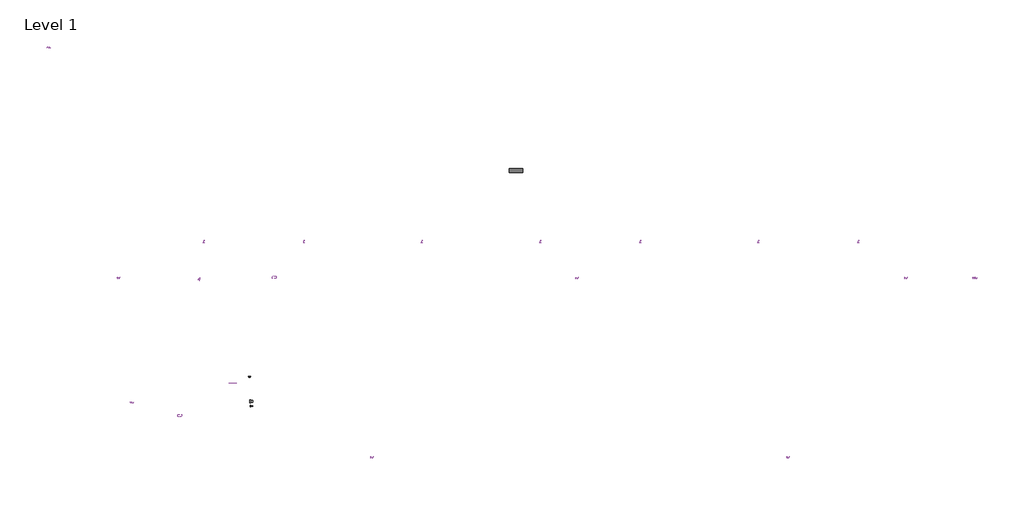
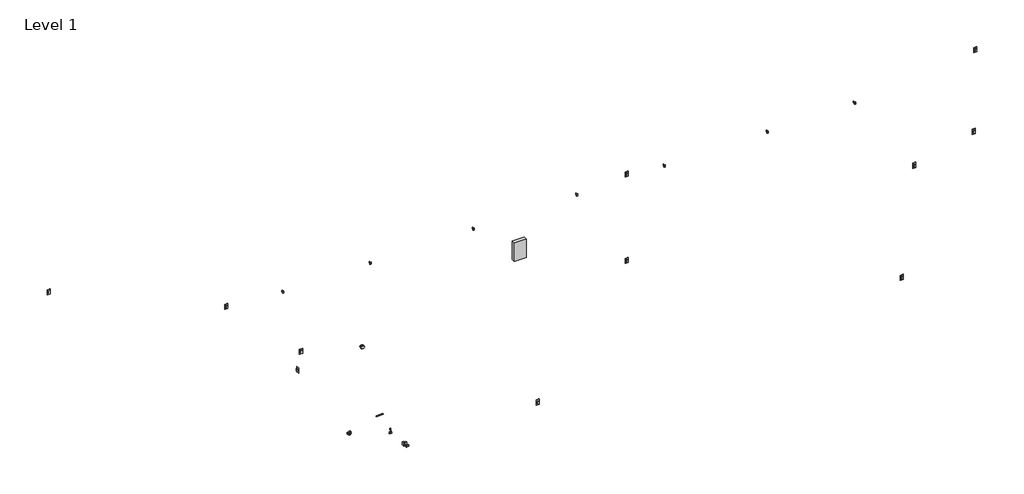
# One storey: 26 proxies.
"""IFC4 building model written with IfcOpenShell, lengths in millimetres."""

import ifcopenshell
import ifcopenshell.guid

model = None  # the IFC model being written
_history = None  # IfcOwnerHistory: only IFC2X3 demands one
_inside = {}  # id of a spatial element -> (the spatial element, [elements in it])
_under = {}  # id of a project, library or spatial element -> (it, [spatial elements below it])
_declared = {}  # id of a project -> (the project, [libraries it declares])
_typed = {}  # id of a type object -> (the type object, [elements of that type])
_made_of = {}  # id of a material, layer set ... -> (it, [elements and type objects made of it])


def new_model(schema):
    """Start an empty IFC model of exactly this schema.

    Asked for "IFC4X3", IfcOpenShell would pick the latest addendum, in which some entities
    have other attributes; the version numbers below select the first issue.
    IFC2X3 requires an IfcOwnerHistory on every rooted entity: one is made here for all.
    """
    global model, _history
    if schema == "IFC4X3":
        model = ifcopenshell.file(schema_version=(4, 3, 0, 0))
    else:
        model = ifcopenshell.file(schema=schema)
    _inside.clear()
    _under.clear()
    _declared.clear()
    _typed.clear()
    _made_of.clear()
    _history = None
    if model.schema == "IFC2X3":
        org = make("IfcOrganization", Name="unknown")
        user = make(
            "IfcPersonAndOrganization",
            ThePerson=make("IfcPerson", FamilyName="unknown"),
            TheOrganization=org,
        )
        app = make(
            "IfcApplication",
            ApplicationDeveloper=org,
            Version="unknown",
            ApplicationFullName="unknown",
            ApplicationIdentifier="unknown",
        )
        _history = make(
            "IfcOwnerHistory",
            OwningUser=user,
            OwningApplication=app,
            ChangeAction="ADDED",
            CreationDate=0,
        )
    return model


def make(cls, **values):
    """One entity of the class cls with the attributes given. An attribute that is None is left unset."""
    return model.create_entity(
        cls, **{name: value for name, value in values.items() if value is not None}
    )


def rooted(cls, **values):
    """An entity with a GlobalId (a new one), such as an element, a storey or a relation."""
    return make(cls, GlobalId=ifcopenshell.guid.new(), OwnerHistory=_history, **values)


def si_unit(unit_type, name, prefix=None):
    """IfcSIUnit, for example si_unit("LENGTHUNIT", "METRE", prefix="MILLI")."""
    return make("IfcSIUnit", UnitType=unit_type, Prefix=prefix, Name=name)


def assignment(units):
    """IfcUnitAssignment: the units of a project."""
    return None if units is None else make("IfcUnitAssignment", Units=units)


def point(xyz):
    """IfcCartesianPoint."""
    return None if xyz is None else make("IfcCartesianPoint", Coordinates=xyz)


def direction(xyz):
    """IfcDirection."""
    return None if xyz is None else make("IfcDirection", DirectionRatios=xyz)


def frame(location, z_axis=None, x_axis=None):
    """IfcAxis2Placement3D, a coordinate frame: its origin and axes. An axis left out is left unset."""
    return make(
        "IfcAxis2Placement3D",
        Location=point(location),
        Axis=direction(z_axis),
        RefDirection=direction(x_axis),
    )


def frame_2d(location, x_axis=None):
    """IfcAxis2Placement2D, a coordinate frame in the plane: its origin and x axis."""
    return make(
        "IfcAxis2Placement2D", Location=point(location), RefDirection=direction(x_axis)
    )


def origin():
    """The frame at (0, 0, 0) with its axes left unset."""
    return frame((0.0, 0.0, 0.0))


def origin_with_axes():
    """The frame at (0, 0, 0) with the z axis (0, 0, 1) and the x axis (1, 0, 0) written out."""
    return frame((0.0, 0.0, 0.0), z_axis=(0.0, 0.0, 1.0), x_axis=(1.0, 0.0, 0.0))


def origin_2d():
    """The frame at (0, 0) in the plane with its x axis left unset."""
    return frame_2d((0.0, 0.0))


def place(relative_to, where):
    """IfcLocalPlacement: puts the frame where relative to a parent placement (None: the world)."""
    return make(
        "IfcLocalPlacement", PlacementRelTo=relative_to, RelativePlacement=where
    )


def context(
    kind, dimensions, precision=None, world=None, true_north=None, identifier=None
):
    """IfcGeometricRepresentationContext, for example the 3D "Model" context."""
    return make(
        "IfcGeometricRepresentationContext",
        ContextIdentifier=identifier,
        ContextType=kind,
        CoordinateSpaceDimension=dimensions,
        Precision=precision,
        WorldCoordinateSystem=world,
        TrueNorth=true_north,
    )


def project(units=None, contexts=None):
    """IfcProject with its units and contexts."""
    return rooted(
        "IfcProject",
        Name="project",
        RepresentationContexts=contexts,
        UnitsInContext=assignment(units),
    )


def spatial(cls, under=None, at=None, **own):
    """A site, building, storey or space (cls), placed at a placement, below another one or the project."""
    s = rooted(cls, ObjectPlacement=at, **own)
    if under is not None:
        _under.setdefault(under.id(), (under, []))[1].append(s)
    return s


def polyline(points):
    """IfcPolyline through the points."""
    return make("IfcPolyline", Points=[point(p) for p in points])


def circle_curve(where, radius):
    """IfcCircle in the frame where."""
    return make("IfcCircle", Position=where, Radius=radius)


def ellipse_curve(where, semi_axis1, semi_axis2):
    """IfcEllipse in the frame where."""
    return make(
        "IfcEllipse", Position=where, SemiAxis1=semi_axis1, SemiAxis2=semi_axis2
    )


def trimmed(basis, trim1, trim2, sense, master):
    """IfcTrimmedCurve: the piece of a basis curve between two trims."""
    return make(
        "IfcTrimmedCurve",
        BasisCurve=basis,
        Trim1=trim1,
        Trim2=trim2,
        SenseAgreement=sense,
        MasterRepresentation=master,
    )


def segment(curve, same_sense, transition):
    """IfcCompositeCurveSegment."""
    return make(
        "IfcCompositeCurveSegment",
        Transition=transition,
        SameSense=same_sense,
        ParentCurve=curve,
    )


def composite_curve(segments, self_intersect=None):
    """IfcCompositeCurve: segments joined end to end."""
    return make("IfcCompositeCurve", Segments=segments, SelfIntersect=self_intersect)


def outline(outer, holes=None, kind="AREA"):
    """IfcArbitraryClosedProfileDef: a profile drawn as a closed curve; with holes, ...WithVoids."""
    if holes is None:
        return make("IfcArbitraryClosedProfileDef", ProfileType=kind, OuterCurve=outer)
    return make(
        "IfcArbitraryProfileDefWithVoids",
        ProfileType=kind,
        OuterCurve=outer,
        InnerCurves=holes,
    )


def extrude(swept, where, along, depth):
    """IfcExtrudedAreaSolid: the profile swept, set in the frame where, extruded along a direction by depth."""
    return make(
        "IfcExtrudedAreaSolid",
        SweptArea=swept,
        Position=where,
        ExtrudedDirection=direction(along),
        Depth=depth,
    )


def shape(context_of_items, identifier, shape_type, items):
    """IfcShapeRepresentation: the items that make up one representation, for example the "Body"."""
    return make(
        "IfcShapeRepresentation",
        ContextOfItems=context_of_items,
        RepresentationIdentifier=identifier,
        RepresentationType=shape_type,
        Items=items,
    )


def source(mapping_origin, context_of_items, identifier, shape_type, items):
    """IfcRepresentationMap: a shape defined once, which mapped items show again and again."""
    return make(
        "IfcRepresentationMap",
        MappingOrigin=mapping_origin,
        MappedRepresentation=shape(context_of_items, identifier, shape_type, items),
    )


def transform(
    local_origin,
    x_axis=None,
    y_axis=None,
    z_axis=None,
    scale=None,
    scale2=None,
    scale3=None,
    uniform=True,
):
    """IfcCartesianTransformationOperator3D, or its non-uniform kind. x_axis, y_axis, z_axis: its Axis1, 2, 3."""
    if uniform:
        return make(
            "IfcCartesianTransformationOperator3D",
            Axis1=direction(x_axis),
            Axis2=direction(y_axis),
            LocalOrigin=point(local_origin),
            Scale=scale,
            Axis3=direction(z_axis),
        )
    return make(
        "IfcCartesianTransformationOperator3DnonUniform",
        Axis1=direction(x_axis),
        Axis2=direction(y_axis),
        LocalOrigin=point(local_origin),
        Scale=scale,
        Axis3=direction(z_axis),
        Scale2=scale2,
        Scale3=scale3,
    )


def mapped(mapping_source, mapping_target):
    """IfcMappedItem: shows the shape of a source again, moved by a transform."""
    return make(
        "IfcMappedItem", MappingSource=mapping_source, MappingTarget=mapping_target
    )


def made_of(thing, what):
    """Note that an element or type object is made of a material, layer set ...; save() writes the relation."""
    if what is not None:
        _made_of.setdefault(what.id(), (what, []))[1].append(thing)
    return thing


def element(
    cls,
    number,
    at=None,
    inside=None,
    cuts=None,
    type_object=None,
    material=None,
    context=None,
    identifier="Body",
    shape_type=None,
    held_by="IfcProductDefinitionShape",
    body=None,
    shapes=None,
    **own,
):
    """One element of the class cls, such as IfcWall. Its Tag is "e" and its number.

    at: its placement. inside: the storey or other place that contains it. cuts: it is an
    opening in that element (IfcRelVoidsElement). A single representation is given by context,
    identifier, shape_type and body (its items); several are given by shapes. held_by: the class
    of the entity that holds the representations. save() writes the other relations.
    """
    e = rooted(cls, Tag="e%d" % number, ObjectPlacement=at, **own)
    if body is not None:
        shapes = [shape(context, identifier, shape_type, body)]
    if shapes is not None:
        e.Representation = make(held_by, Representations=shapes)
    if inside is not None:
        _inside.setdefault(inside.id(), (inside, []))[1].append(e)
    if cuts is not None:
        rooted(
            "IfcRelVoidsElement", RelatingBuildingElement=cuts, RelatedOpeningElement=e
        )
    if type_object is not None:
        _typed.setdefault(type_object.id(), (type_object, []))[1].append(e)
    return made_of(e, material)


def aggregate(whole, parts):
    """IfcRelAggregates: a whole, such as a stair, and the parts it consists of."""
    return rooted("IfcRelAggregates", RelatingObject=whole, RelatedObjects=parts)


def save(model, path):
    """Write the relations noted so far, then the file.

    IfcRelAggregates (storeys below a building ...), IfcRelContainedInSpatialStructure (elements
    in a storey), IfcRelDefinesByType, IfcRelAssociatesMaterial and IfcRelDeclares: one each for
    every whole, place, type object, material and project.
    """
    for whole, parts in _under.values():
        aggregate(whole, parts)
    for where, things in _inside.values():
        rooted(
            "IfcRelContainedInSpatialStructure",
            RelatedElements=things,
            RelatingStructure=where,
        )
    for kind, things in _typed.values():
        rooted("IfcRelDefinesByType", RelatedObjects=things, RelatingType=kind)
    for what, things in _made_of.values():
        rooted("IfcRelAssociatesMaterial", RelatedObjects=things, RelatingMaterial=what)
    for by, libraries in _declared.values():
        rooted("IfcRelDeclares", RelatingContext=by, RelatedDefinitions=libraries)
    model.write(path)


def plane_surface(at):
    """IfcPlane: the flat surface through the origin of the frame at, square to its z axis."""
    return make("IfcPlane", Position=at)


def cylinder_surface(at, radius):
    """IfcCylindricalSurface: all points at the distance radius from the z axis of the frame at."""
    return make("IfcCylindricalSurface", Position=at, Radius=radius)


def revolved_surface(curve, axis_point, axis_direction):
    """IfcSurfaceOfRevolution: the curve turned about the line through axis_point along axis_direction."""
    return make(
        "IfcSurfaceOfRevolution",
        SweptCurve=make("IfcArbitraryOpenProfileDef", ProfileType="CURVE", Curve=curve),
        AxisPosition=make("IfcAxis1Placement", Location=point(axis_point), Axis=direction(axis_direction)),
    )


def advanced_brep(points, edges, surfaces, faces):
    """IfcAdvancedBrep: a solid bounded by faces that lie on surfaces and meet in shared edges.

    An edge is (start, end): straight between two places in points (the first is 0);
    or (start, end, curve); or (start, end, curve, False) where it runs against its curve.
    A face is (place in surfaces, loops), or (place, loops, False) where it looks against
    its surface's normal. A loop lists edges by number (the first is 1), with a minus sign
    where the edge is run from its end to its start. The first loop is the outer one.
    """
    corners = [point(p) for p in points]
    vertices = [make("IfcVertexPoint", VertexGeometry=c) for c in corners]
    made = []
    for start, end, *more in edges:
        made.append(
            make(
                "IfcEdgeCurve",
                EdgeStart=vertices[start],
                EdgeEnd=vertices[end],
                EdgeGeometry=more[0] if more else make("IfcPolyline", Points=[corners[start], corners[end]]),
                SameSense=more[1] if len(more) > 1 else True,
            )
        )
    hull = []
    for where, loops, *sense in faces:
        bounds = []
        for j, loop in enumerate(loops):
            ring = [make("IfcOrientedEdge", EdgeElement=made[abs(k) - 1], Orientation=k > 0) for k in loop]
            bounds.append(
                make(
                    "IfcFaceOuterBound" if j == 0 else "IfcFaceBound",
                    Bound=make("IfcEdgeLoop", EdgeList=ring),
                    Orientation=True,
                )
            )
        hull.append(make("IfcAdvancedFace", Bounds=bounds, FaceSurface=surfaces[where], SameSense=sense[0] if sense else True))
    return make("IfcAdvancedBrep", Outer=make("IfcClosedShell", CfsFaces=hull))


def access_card_reader_standard_2fd2a6f3(model_context):
    return source(origin(), model_context, "Body", "SweptSolid", [
        extrude(outline(polyline([(23.0, -85.0), (-23.0, -85.0), (-23.0, 0.0), (23.0, 0.0), (23.0, -85.0)])), origin_with_axes(), (0.0, 0.0, 1.0), 19.0),
        extrude(outline(polyline([(10.5, -72.5), (-10.5, -72.5), (-10.5, -12.5), (10.5, -12.5), (10.5, -72.5)])), frame((0.0, 0.0, -82.0), z_axis=(0.0, 0.0, 1.0), x_axis=(1.0, 0.0, 0.0)), (0.0, 0.0, 1.0), 82.0),
    ])


def bell_standard_b2399fa3(model_context):
    return source(origin(), model_context, "Body", "SweptSolid", [
        extrude(outline(polyline([(46.5, -145.0), (-46.5, -145.0), (-46.5, 0.0), (46.5, 0.0), (46.5, -145.0)])), origin_with_axes(), (0.0, 0.0, 1.0), 39.0),
        extrude(outline(polyline([(34.0, -132.5), (-34.0, -132.5), (-34.0, -12.5), (34.0, -12.5), (34.0, -132.5)])), frame((0.0, 0.0, -84.0286528), z_axis=(0.0, 0.0, 1.0), x_axis=(1.0, 0.0, 0.0)), (0.0, 0.0, 1.0), 84.0286528),
    ])


def door_lock_magnetic_standard_083446a8(model_context):
    return source(origin(), model_context, "Body", "SweptSolid", [
        extrude(outline(polyline([(142.5, -40.0), (-142.5, -40.0), (-142.5, 0.0), (142.5, 0.0), (142.5, -40.0)])), origin_with_axes(), (0.0, 0.0, 1.0), 8.0),
        extrude(outline(polyline([(130.0, -27.5), (-130.0, -27.5), (-130.0, -12.5), (130.0, -12.5), (130.0, -27.5)])), frame((0.0, 0.0, -20.0), z_axis=(0.0, 0.0, 1.0), x_axis=(1.0, 0.0, 0.0)), (0.0, 0.0, 1.0), 20.0),
    ])


def keypad_standard_b9346bd5(model_context):
    return source(origin(), model_context, "Body", "SweptSolid", [
        extrude(outline(polyline([(19.0, -60.0), (-19.0, -60.0), (-19.0, 0.0), (19.0, 0.0), (19.0, -60.0)])), origin_with_axes(), (0.0, 0.0, 1.0), 8.0),
        extrude(outline(polyline([(6.5, -47.5), (-6.5, -47.5), (-6.5, -12.5), (6.5, -12.5), (6.5, -47.5)])), frame((0.0, 0.0, -14.0), z_axis=(0.0, 0.0, 1.0), x_axis=(1.0, 0.0, 0.0)), (0.0, 0.0, 1.0), 14.0),
        extrude(outline(composite_curve([segment(trimmed(circle_curve(frame_2d((-13.0, -17.8125)), 3.25), [point((-9.75, -17.8125))], [point((-16.25, -17.8125))], False, "CARTESIAN"), True, "CONTINUOUS"), segment(trimmed(circle_curve(frame_2d((-13.0, -17.8125)), 3.25), [point((-16.25, -17.8125))], [point((-9.75, -17.8125))], False, "CARTESIAN"), True, "CONTINUOUS")], self_intersect=False)), frame((0.0, 0.0, 8.0), z_axis=(0.0, 0.0, 1.0), x_axis=(1.0, 0.0, 0.0)), (0.0, 0.0, 1.0), 1.0),
        extrude(outline(composite_curve([segment(trimmed(circle_curve(frame_2d((-13.0, -29.8125)), 3.25), [point((-9.75, -29.8125))], [point((-16.25, -29.8125))], False, "CARTESIAN"), True, "CONTINUOUS"), segment(trimmed(circle_curve(frame_2d((-13.0, -29.8125)), 3.25), [point((-16.25, -29.8125))], [point((-9.75, -29.8125))], False, "CARTESIAN"), True, "CONTINUOUS")], self_intersect=False)), frame((0.0, 0.0, 8.0), z_axis=(0.0, 0.0, 1.0), x_axis=(1.0, 0.0, 0.0)), (0.0, 0.0, 1.0), 1.0),
        extrude(outline(composite_curve([segment(trimmed(circle_curve(frame_2d((-13.0, -41.8125)), 3.25), [point((-9.75, -41.8125))], [point((-16.25, -41.8125))], False, "CARTESIAN"), True, "CONTINUOUS"), segment(trimmed(circle_curve(frame_2d((-13.0, -41.8125)), 3.25), [point((-16.25, -41.8125))], [point((-9.75, -41.8125))], False, "CARTESIAN"), True, "CONTINUOUS")], self_intersect=False)), frame((0.0, 0.0, 8.0), z_axis=(0.0, 0.0, 1.0), x_axis=(1.0, 0.0, 0.0)), (0.0, 0.0, 1.0), 1.0),
        extrude(outline(composite_curve([segment(trimmed(circle_curve(frame_2d((-13.0, -53.8125)), 3.25), [point((-9.75, -53.8125))], [point((-16.25, -53.8125))], False, "CARTESIAN"), True, "CONTINUOUS"), segment(trimmed(circle_curve(frame_2d((-13.0, -53.8125)), 3.25), [point((-16.25, -53.8125))], [point((-9.75, -53.8125))], False, "CARTESIAN"), True, "CONTINUOUS")], self_intersect=False)), frame((0.0, 0.0, 8.0), z_axis=(0.0, 0.0, 1.0), x_axis=(1.0, 0.0, 0.0)), (0.0, 0.0, 1.0), 1.0),
        extrude(outline(composite_curve([segment(trimmed(circle_curve(frame_2d((13.0, -53.8125)), 3.25), [point((16.25, -53.8125))], [point((9.75, -53.8125))], False, "CARTESIAN"), True, "CONTINUOUS"), segment(trimmed(circle_curve(frame_2d((13.0, -53.8125)), 3.25), [point((9.75, -53.8125))], [point((16.25, -53.8125))], False, "CARTESIAN"), True, "CONTINUOUS")], self_intersect=False)), frame((0.0, 0.0, 8.0), z_axis=(0.0, 0.0, 1.0), x_axis=(1.0, 0.0, 0.0)), (0.0, 0.0, 1.0), 1.0),
        extrude(outline(composite_curve([segment(trimmed(circle_curve(frame_2d((0.0, -53.8125)), 3.25), [point((3.25, -53.8125))], [point((-3.25, -53.8125))], False, "CARTESIAN"), True, "CONTINUOUS"), segment(trimmed(circle_curve(frame_2d((0.0, -53.8125)), 3.25), [point((-3.25, -53.8125))], [point((3.25, -53.8125))], False, "CARTESIAN"), True, "CONTINUOUS")], self_intersect=False)), frame((0.0, 0.0, 8.0), z_axis=(0.0, 0.0, 1.0), x_axis=(1.0, 0.0, 0.0)), (0.0, 0.0, 1.0), 1.0),
        extrude(outline(composite_curve([segment(trimmed(circle_curve(frame_2d((0.0, -41.8125)), 3.25), [point((3.25, -41.8125))], [point((-3.25, -41.8125))], False, "CARTESIAN"), True, "CONTINUOUS"), segment(trimmed(circle_curve(frame_2d((0.0, -41.8125)), 3.25), [point((-3.25, -41.8125))], [point((3.25, -41.8125))], False, "CARTESIAN"), True, "CONTINUOUS")], self_intersect=False)), frame((0.0, 0.0, 8.0), z_axis=(0.0, 0.0, 1.0), x_axis=(1.0, 0.0, 0.0)), (0.0, 0.0, 1.0), 1.0),
        extrude(outline(composite_curve([segment(trimmed(circle_curve(frame_2d((0.0, -29.8125)), 3.25), [point((3.25, -29.8125))], [point((-3.25, -29.8125))], False, "CARTESIAN"), True, "CONTINUOUS"), segment(trimmed(circle_curve(frame_2d((0.0, -29.8125)), 3.25), [point((-3.25, -29.8125))], [point((3.25, -29.8125))], False, "CARTESIAN"), True, "CONTINUOUS")], self_intersect=False)), frame((0.0, 0.0, 8.0), z_axis=(0.0, 0.0, 1.0), x_axis=(1.0, 0.0, 0.0)), (0.0, 0.0, 1.0), 1.0),
        extrude(outline(composite_curve([segment(trimmed(circle_curve(frame_2d((0.0, -17.8125)), 3.25), [point((3.25, -17.8125))], [point((-3.25, -17.8125))], False, "CARTESIAN"), True, "CONTINUOUS"), segment(trimmed(circle_curve(frame_2d((0.0, -17.8125)), 3.25), [point((-3.25, -17.8125))], [point((3.25, -17.8125))], False, "CARTESIAN"), True, "CONTINUOUS")], self_intersect=False)), frame((0.0, 0.0, 8.0), z_axis=(0.0, 0.0, 1.0), x_axis=(1.0, 0.0, 0.0)), (0.0, 0.0, 1.0), 1.0),
        extrude(outline(composite_curve([segment(trimmed(circle_curve(frame_2d((13.0, -17.8125)), 3.25), [point((16.25, -17.8125))], [point((9.75, -17.8125))], False, "CARTESIAN"), True, "CONTINUOUS"), segment(trimmed(circle_curve(frame_2d((13.0, -17.8125)), 3.25), [point((9.75, -17.8125))], [point((16.25, -17.8125))], False, "CARTESIAN"), True, "CONTINUOUS")], self_intersect=False)), frame((0.0, 0.0, 8.0), z_axis=(0.0, 0.0, 1.0), x_axis=(1.0, 0.0, 0.0)), (0.0, 0.0, 1.0), 1.0),
        extrude(outline(composite_curve([segment(trimmed(circle_curve(frame_2d((13.0, -29.8125)), 3.25), [point((16.25, -29.8125))], [point((9.75, -29.8125))], False, "CARTESIAN"), True, "CONTINUOUS"), segment(trimmed(circle_curve(frame_2d((13.0, -29.8125)), 3.25), [point((9.75, -29.8125))], [point((16.25, -29.8125))], False, "CARTESIAN"), True, "CONTINUOUS")], self_intersect=False)), frame((0.0, 0.0, 8.0), z_axis=(0.0, 0.0, 1.0), x_axis=(1.0, 0.0, 0.0)), (0.0, 0.0, 1.0), 1.0),
        extrude(outline(composite_curve([segment(trimmed(circle_curve(frame_2d((13.0, -41.8125)), 3.25), [point((16.25, -41.8125))], [point((9.75, -41.8125))], False, "CARTESIAN"), True, "CONTINUOUS"), segment(trimmed(circle_curve(frame_2d((13.0, -41.8125)), 3.25), [point((9.75, -41.8125))], [point((16.25, -41.8125))], False, "CARTESIAN"), True, "CONTINUOUS")], self_intersect=False)), frame((0.0, 0.0, 8.0), z_axis=(0.0, 0.0, 1.0), x_axis=(1.0, 0.0, 0.0)), (0.0, 0.0, 1.0), 1.0),
        extrude(outline(polyline([(16.0429892, -9.21875), (-16.25, -9.21875), (-16.25, -1.2800214), (16.0429892, -1.2800214), (16.0429892, -9.21875)])), frame((0.0, 0.0, 8.0), z_axis=(0.0, 0.0, 1.0), x_axis=(1.0, 0.0, 0.0)), (0.0, 0.0, 1.0), 1.0),
    ])


def release_button_standard_0a205331(model_context):
    return source(origin(), model_context, "Body", "SweptSolid", [
        extrude(outline(polyline([(42.5, -85.0), (-42.5, -85.0), (-42.5, 0.0), (42.5, 0.0), (42.5, -85.0)])), origin_with_axes(), (0.0, 0.0, 1.0), 8.0),
        extrude(outline(polyline([(30.0, -72.5), (-30.0, -72.5), (-30.0, -12.5), (30.0, -12.5), (30.0, -72.5)])), frame((0.0, 0.0, -33.0), z_axis=(0.0, 0.0, 1.0), x_axis=(1.0, 0.0, 0.0)), (0.0, 0.0, 1.0), 33.0),
    ])


def security_panel_225_a_071659d5(model_context):
    return source(origin(), model_context, "Body", "SweptSolid", [
        extrude(outline(polyline([(250.0, -11.6), (250.0, -826.6), (-250.0, -826.6), (-250.0, -11.6), (250.0, -11.6)])), frame((0.0, 0.0, -150.0), z_axis=(0.0, 0.0, 1.0), x_axis=(1.0, 0.0, 0.0)), (0.0, 0.0, 1.0), 150.0),
    ])


def standard_da8f596e(model_context):
    return source(origin(), model_context, "Body", "SolidModel", [
        extrude(outline(polyline([(-50.8099209, -85.0), (-52.6934767, -85.0), (-52.6934767, -80.0), (-50.8099209, -80.0), (-50.8099209, -85.0)])), frame((0.0, 0.0, 4.6605901), z_axis=(0.0, 0.0, 1.0), x_axis=(1.0, 0.0, 0.0)), (0.0, 0.0, 1.0), 15.0684465),
        extrude(outline(polyline([(4.6605901, -47.0428093), (4.6605901, -45.1592535), (16.6020397, -45.1592535), (4.6605901, -37.2865788), (4.6605901, -35.2705855), (19.7290366, -35.2705855), (19.7290366, -37.1541413), (7.7912659, -37.1541413), (19.7290366, -45.026816), (19.7290366, -47.0428093), (4.6605901, -47.0428093)])), frame((0.0, -85.0, 0.0), z_axis=(0.0, 1.0, 0.0), x_axis=(0.0, 0.0, 1.0)), (0.0, 0.0, 1.0), 5.0),
        extrude(outline(polyline([(4.6605901, -28.2072512), (4.6605901, -26.3236953), (17.8454808, -26.3236953), (17.8454808, -21.3793613), (19.7290366, -21.3793613), (19.7290366, -33.1515852), (17.8454808, -33.1515852), (17.8454808, -28.2072512), (4.6605901, -28.2072512)])), frame((0.0, -85.0, 0.0), z_axis=(0.0, 1.0, 0.0), x_axis=(0.0, 0.0, 1.0)), (0.0, 0.0, 1.0), 5.0),
        extrude(outline(polyline([(4.6605901, -19.260361), (4.6605901, -17.3768052), (11.2530355, -17.3768052), (9.8514051, -12.1197715), (7.7839082, -10.7034258), (4.6605901, -8.7426148), (4.6605901, -6.5537169), (8.7440802, -9.0663509), (11.4884799, -11.6635978), (12.8901103, -8.5090097), (15.6050795, -7.4881372), (17.8841084, -8.1043395), (19.322527, -9.7524509), (19.7290366, -12.7672438), (19.7290366, -19.260361), (4.6605901, -19.260361)]), holes=[polyline([(13.1365913, -17.3768052), (17.8454808, -17.3768052), (17.8454808, -12.6863098), (17.1943297, -10.1681575), (13.4033057, -11.0106073), (13.1365913, -13.1608775), (13.1365913, -17.3768052)])]), frame((0.0, -85.0, 0.0), z_axis=(0.0, 1.0, 0.0), x_axis=(0.0, 0.0, 1.0)), (0.0, 0.0, 1.0), 5.0),
        extrude(outline(polyline([(19.7290366, 5.6967535), (11.1022038, 5.6967535), (7.298304, 4.7439392), (6.3087014, 1.5544023), (6.809021, -0.6602474), (8.2308849, -1.9367979), (11.1022038, -2.3083587), (19.7290366, -2.3083587), (19.7290366, -4.1919145), (11.0359851, -4.1919145), (7.2633552, -3.619858), (5.153552, -1.7105504), (4.4251456, 1.7309856), (5.2620772, 5.2258646), (7.4325809, 7.0689534), (11.0359851, 7.5803093), (19.7290366, 7.5803093), (19.7290366, 5.6967535)])), frame((0.0, -85.0, 0.0), z_axis=(0.0, 1.0, 0.0), x_axis=(0.0, 0.0, 1.0)), (0.0, 0.0, 1.0), 5.0),
        extrude(outline(polyline([(4.6605901, 10.876532), (4.6605901, 16.3248644), (4.9181075, 18.7473673), (5.674105, 20.5481497), (7.0407866, 21.9240283), (9.2352027, 22.9540979), (12.2757474, 23.3550893), (15.858918, 22.7627993), (18.434092, 20.9785716), (19.5119862, 18.763922), (19.7290366, 16.0747046), (19.7290366, 10.876532), (4.6605901, 10.876532)]), holes=[polyline([(6.5441459, 12.7600878), (17.8454808, 12.7600878), (17.8454808, 16.0415952), (17.5438176, 18.7124185), (15.8736333, 20.6677113), (12.305178, 21.4715335), (9.4559319, 21.0613451), (7.585252, 19.9153926), (6.8163786, 18.5174411), (6.5441459, 16.0930987), (6.5441459, 12.7600878)])]), frame((0.0, -85.0, 0.0), z_axis=(0.0, 1.0, 0.0), x_axis=(0.0, 0.0, 1.0)), (0.0, 0.0, 1.0), 5.0),
        extrude(outline(polyline([(4.6605901, 25.9449785), (4.6605901, 37.010869), (6.5441459, 37.010869), (6.5441459, 27.8285344), (11.4884799, 27.8285344), (11.4884799, 36.3045355), (13.3720357, 36.3045355), (13.3720357, 27.8285344), (17.8454808, 27.8285344), (17.8454808, 36.7754245), (19.7290366, 36.7754245), (19.7290366, 25.9449785), (4.6605901, 25.9449785)])), frame((0.0, -85.0, 0.0), z_axis=(0.0, 1.0, 0.0), x_axis=(0.0, 0.0, 1.0)), (0.0, 0.0, 1.0), 5.0),
        extrude(outline(polyline([(4.6605901, 39.8362027), (4.6605901, 41.7197585), (11.2530355, 41.7197585), (9.8514051, 46.9767922), (7.7839082, 48.3931379), (4.6605901, 50.3539489), (4.6605901, 52.5428468), (8.7440802, 50.0302128), (11.4884799, 47.4329659), (12.8901103, 50.587554), (15.6050795, 51.6084265), (17.8841084, 50.9922242), (19.322527, 49.3441128), (19.7290366, 46.3293199), (19.7290366, 39.8362027), (4.6605901, 39.8362027)]), holes=[polyline([(13.1365913, 41.7197585), (17.8454808, 41.7197585), (17.8454808, 46.4102539), (17.1943297, 48.9284062), (13.4033057, 48.0859564), (13.1365913, 45.9356862), (13.1365913, 41.7197585)])]), frame((0.0, -85.0, 0.0), z_axis=(0.0, 1.0, 0.0), x_axis=(0.0, 0.0, 1.0)), (0.0, 0.0, 1.0), 5.0),
        extrude(outline(polyline([(-8.4558541, -53.6352547), (-11.3326913, -52.8222354), (-13.23832, -50.6940381), (-13.8710771, -47.3297573), (-13.2843053, -44.4805112), (-11.6398728, -42.5380943), (-9.3865955, -41.8630308), (-7.2565588, -42.4498026), (-5.7298485, -44.2726579), (-4.7843918, -47.6056688), (-2.4262682, -51.2808099), (-0.8627697, -50.4346813), (-0.2152974, -47.7381063), (-0.8701273, -45.0488889), (-2.8051866, -43.9820311), (-2.8051866, -42.0984753), (-0.447063, -42.8452757), (1.1311507, -44.8318385), (1.6682584, -47.8116827), (1.155063, -50.603907), (-0.3495743, -52.5113752), (-2.4814505, -53.1643657), (-4.3539698, -52.636455), (-5.7556002, -51.034329), (-6.6845023, -48.0820759), (-11.6435516, -45.435165), (-11.9875212, -47.4033337), (-11.533187, -49.6621291), (-10.3412493, -51.1446935), (-8.4558541, -51.7516988), (-8.4558541, -53.6352547)])), frame((0.0, -85.0, 0.0), z_axis=(0.0, 1.0, 0.0), x_axis=(0.0, 0.0, 1.0)), (0.0, 0.0, 1.0), 5.0),
        extrude(outline(polyline([(-13.6356326, -39.0376971), (-13.6356326, -27.9718067), (-11.7520768, -27.9718067), (-11.7520768, -37.1541413), (-6.8077427, -37.1541413), (-6.8077427, -28.6781401), (-4.9241869, -28.6781401), (-4.9241869, -37.1541413), (-0.4507419, -37.1541413), (-0.4507419, -28.2072512), (1.4328139, -28.2072512), (1.4328139, -39.0376971), (-13.6356326, -39.0376971)])), frame((0.0, -85.0, 0.0), z_axis=(0.0, 1.0, 0.0), x_axis=(0.0, 0.0, 1.0)), (0.0, 0.0, 1.0), 5.0),
        extrude(outline(polyline([(-8.2792707, -14.5514715), (-11.053101, -16.1499188), (-11.9875212, -19.0322742), (-11.3014213, -21.6313605), (-9.2284063, -23.4008729), (-5.9836871, -23.9692506), (-3.1841051, -23.4891646), (-1.020959, -21.8244985), (-0.2152974, -18.8777638), (-0.9418643, -16.3320203), (-3.2576815, -14.786916), (-2.8088655, -12.9033602), (0.4947149, -15.0315575), (1.6682584, -18.8041874), (0.7614293, -22.4241462), (-1.8928393, -24.9606925), (-5.9873659, -25.8528064), (-10.0156737, -25.0636995), (-12.8814745, -22.764437), (-13.8710771, -18.8446544), (-12.5632566, -14.9009594), (-8.764875, -12.6679157), (-8.2792707, -14.5514715)])), frame((0.0, -85.0, 0.0), z_axis=(0.0, 1.0, 0.0), x_axis=(0.0, 0.0, 1.0)), (0.0, 0.0, 1.0), 5.0),
        extrude(outline(polyline([(1.4328139, -0.1893584), (-7.1940188, -0.1893584), (-10.9979187, -1.1421728), (-11.9875212, -4.3317097), (-11.4872017, -6.5463593), (-10.0653378, -7.8229098), (-7.1940188, -8.1944706), (1.4328139, -8.1944706), (1.4328139, -10.0780264), (-7.2602376, -10.0780264), (-11.0328675, -9.5059699), (-13.1426707, -7.5966624), (-13.8710771, -4.1551263), (-13.0341455, -0.6602474), (-10.8636417, 1.1828414), (-7.2602376, 1.6941974), (1.4328139, 1.6941974), (1.4328139, -0.1893584)])), frame((0.0, -85.0, 0.0), z_axis=(0.0, 1.0, 0.0), x_axis=(0.0, 0.0, 1.0)), (0.0, 0.0, 1.0), 5.0),
        extrude(outline(polyline([(-13.6356326, 4.9904201), (-13.6356326, 6.8739759), (-7.0431872, 6.8739759), (-8.4448176, 12.1310096), (-10.5123144, 13.5473553), (-13.6356326, 15.5081663), (-13.6356326, 17.6970642), (-9.5521424, 15.1844302), (-6.8077427, 12.5871833), (-5.4061123, 15.7417714), (-2.6911432, 16.7626439), (-0.4121143, 16.1464416), (1.0263043, 14.4983303), (1.4328139, 11.4835373), (1.4328139, 4.9904201), (-13.6356326, 4.9904201)]), holes=[polyline([(-5.1596314, 6.8739759), (-0.4507419, 6.8739759), (-0.4507419, 11.5644713), (-1.101893, 14.0826236), (-4.892917, 13.2401738), (-5.1596314, 11.0899036), (-5.1596314, 6.8739759)])]), frame((0.0, -85.0, 0.0), z_axis=(0.0, 1.0, 0.0), x_axis=(0.0, 0.0, 1.0)), (0.0, 0.0, 1.0), 5.0),
        extrude(outline(polyline([(22.1778669, -85.0), (20.2943111, -85.0), (20.2943111, -80.0), (22.1778669, -80.0), (22.1778669, -85.0)])), frame((0.0, 0.0, -13.6356326), z_axis=(0.0, 0.0, 1.0), x_axis=(1.0, 0.0, 0.0)), (0.0, 0.0, 1.0), 15.0684465),
        extrude(outline(polyline([(-13.6356326, 29.7120902), (-13.6356326, 31.595646), (-0.4507419, 31.595646), (-0.4507419, 36.53998), (1.4328139, 36.53998), (1.4328139, 24.7677562), (-0.4507419, 24.7677562), (-0.4507419, 29.7120902), (-13.6356326, 29.7120902)])), frame((0.0, -85.0, 0.0), z_axis=(0.0, 1.0, 0.0), x_axis=(0.0, 0.0, 1.0)), (0.0, 0.0, 1.0), 5.0),
        extrude(outline(polyline([(-13.6356326, 42.8969809), (-13.6356326, 44.7805367), (-7.25288, 44.7805367), (1.4328139, 50.6666486), (1.4328139, 48.4446414), (-3.0369523, 45.5935559), (-5.5716592, 43.9822328), (-3.206178, 42.3745884), (1.4328139, 39.2328762), (1.4328139, 37.010869), (-7.25288, 42.8969809), (-13.6356326, 42.8969809)])), frame((0.0, -85.0, 0.0), z_axis=(0.0, 1.0, 0.0), x_axis=(0.0, 0.0, 1.0)), (0.0, 0.0, 1.0), 5.0),
        extrude(outline(polyline([(-31.9318553, -36.5544936), (-31.9318553, -34.564252), (-27.2229657, -32.8425643), (-27.2229657, -26.636395), (-31.9318553, -24.9110285), (-31.9318553, -22.9207869), (-16.8634087, -28.9356575), (-16.8634087, -30.539623), (-31.9318553, -36.5544936)]), holes=[polyline([(-25.3394099, -32.1509461), (-21.3111021, -30.6757393), (-18.7469645, -29.7376403), (-21.6348382, -28.6818189), (-25.3394099, -27.3243344), (-25.3394099, -32.1509461)])]), frame((0.0, -85.0, 0.0), z_axis=(0.0, 1.0, 0.0), x_axis=(0.0, 0.0, 1.0)), (0.0, 0.0, 1.0), 5.0),
        extrude(outline(polyline([(-31.9318553, -20.9084724), (-31.9318553, -11.4906933), (-30.0482994, -11.4906933), (-30.0482994, -19.0249166), (-16.8634087, -19.0249166), (-16.8634087, -20.9084724), (-31.9318553, -20.9084724)])), frame((0.0, -85.0, 0.0), z_axis=(0.0, 1.0, 0.0), x_axis=(0.0, 0.0, 1.0)), (0.0, 0.0, 1.0), 5.0),
        extrude(outline(polyline([(-31.9318553, -11.1264901), (-31.9318553, -9.1362485), (-27.2229657, -7.4145608), (-27.2229657, -1.2083915), (-31.9318553, 0.516975), (-31.9318553, 2.5072166), (-16.8634087, -3.507654), (-16.8634087, -5.1116195), (-31.9318553, -11.1264901)]), holes=[polyline([(-25.3394099, -6.7229426), (-21.3111021, -5.2477358), (-18.7469645, -4.3096367), (-21.6348382, -3.2538154), (-25.3394099, -1.8963309), (-25.3394099, -6.7229426)])]), frame((0.0, -85.0, 0.0), z_axis=(0.0, 1.0, 0.0), x_axis=(0.0, 0.0, 1.0)), (0.0, 0.0, 1.0), 5.0),
        extrude(outline(polyline([(-31.9318553, 4.5195311), (-31.9318553, 6.403087), (-25.3394099, 6.403087), (-26.7410403, 11.6601207), (-28.8085371, 13.0764663), (-31.9318553, 15.0372774), (-31.9318553, 17.2261753), (-27.8483651, 14.7135412), (-25.1039654, 12.1162943), (-23.702335, 15.2708824), (-20.9873659, 16.291755), (-18.7083369, 15.6755526), (-17.2699183, 14.0274413), (-16.8634087, 11.0126484), (-16.8634087, 4.5195311), (-31.9318553, 4.5195311)]), holes=[polyline([(-23.4558541, 6.403087), (-18.7469645, 6.403087), (-18.7469645, 11.0935824), (-19.3981157, 13.6117347), (-23.1891396, 12.7692849), (-23.4558541, 10.6190146), (-23.4558541, 6.403087)])]), frame((0.0, -85.0, 0.0), z_axis=(0.0, 1.0, 0.0), x_axis=(0.0, 0.0, 1.0)), (0.0, 0.0, 1.0), 5.0),
        extrude(outline(polyline([(-31.9318553, 19.5879777), (-31.9318553, 21.4715335), (-18.7469645, 21.4715335), (-31.9318553, 25.2570392), (-31.9318553, 27.8101403), (-18.7469645, 31.595646), (-31.9318553, 31.595646), (-31.9318553, 33.4792018), (-16.8634087, 33.4792018), (-16.8634087, 30.2381614), (-27.3002209, 27.2068138), (-29.7024904, 26.5335897), (-27.4841619, 25.9118692), (-16.8634087, 22.829018), (-16.8634087, 19.5879777), (-31.9318553, 19.5879777)])), frame((0.0, -85.0, 0.0), z_axis=(0.0, 1.0, 0.0), x_axis=(0.0, 0.0, 1.0)), (0.0, 0.0, 1.0), 5.0),
        extrude(outline(composite_curve([segment(polyline([(38.0, 64.6606526), (38.0, -64.6606526)]), True, "CONTINUOUS"), segment(trimmed(circle_curve(origin_2d(), 75.0), [point((38.0, -64.6606526))], [point((0.0, -75.0))], False, "CARTESIAN"), True, "CONTINUOUS"), segment(trimmed(circle_curve(origin_2d(), 75.0), [point((0.0, -75.0))], [point((-56.0, -49.8898787))], False, "CARTESIAN"), True, "CONTINUOUS"), segment(polyline([(-56.0, -49.8898787), (-56.0, 49.8898787)]), True, "CONTINUOUS"), segment(trimmed(circle_curve(origin_2d(), 75.0), [point((-56.0, 49.8898787))], [point((0.0, 75.0))], False, "CARTESIAN"), True, "CONTINUOUS"), segment(trimmed(circle_curve(origin_2d(), 75.0), [point((0.0, 75.0))], [point((38.0, 64.6606526))], False, "CARTESIAN"), True, "CONTINUOUS")], self_intersect=False)), frame((0.0, -30.0, 0.0), z_axis=(0.0, 1.0, 0.0), x_axis=(0.0, 0.0, 1.0)), (0.0, 0.0, 1.0), 30.0),
        advanced_brep(
        [(-65.0, -80.0, 0.0), (65.0, -80.0, 0.0), (0.0, -80.0, 0.0), (-75.0, -70.0, 0.0), (75.0, -70.0, 0.0), (-75.0, -30.0, 0.0), (75.0, -30.0, 0.0), (0.0, -30.0, 0.0)],
        [
            (0, 1, circle_curve(frame((0.0, -80.0, 0.0), z_axis=(0.0, -1.0, 0.0), x_axis=(1.0, 0.0, 0.0)), 65.0)),
            (1, 2),
            (2, 0),
            (1, 0, circle_curve(frame((0.0, -80.0, 0.0), z_axis=(0.0, -1.0, 0.0), x_axis=(1.0, 0.0, 0.0)), 65.0)),
            (3, 4, circle_curve(frame((0.0, -70.0, 0.0), z_axis=(0.0, -1.0, 0.0), x_axis=(1.0, 0.0, 0.0)), 75.0)),
            (4, 1, circle_curve(frame((65.0, -70.0, 0.0), z_axis=(0.0, 0.0, -1.0), x_axis=(-1.0, 0.0, 0.0)), 10.0)),
            (0, 3, circle_curve(frame((-65.0, -70.0, 0.0), z_axis=(0.0, 0.0, -1.0), x_axis=(1.0, 0.0, 0.0)), 10.0)),
            (4, 3, circle_curve(frame((0.0, -70.0, 0.0), z_axis=(0.0, -1.0, 0.0), x_axis=(1.0, 0.0, 0.0)), 75.0)),
            (5, 6, circle_curve(frame((0.0, -30.0, 0.0), z_axis=(0.0, -1.0, 0.0), x_axis=(1.0, 0.0, 0.0)), 75.0)),
            (6, 4),
            (3, 5),
            (6, 5, circle_curve(frame((0.0, -30.0, 0.0), z_axis=(0.0, -1.0, 0.0), x_axis=(1.0, 0.0, 0.0)), 75.0)),
            (7, 6),
            (5, 7),
        ],
        [
            plane_surface(frame((0.0, -80.0, 0.0), z_axis=(0.0, -1.0, 0.0), x_axis=(1.0, 0.0, 0.0))),
            revolved_surface(trimmed(ellipse_curve(frame((65.0, -70.0, 0.0), z_axis=(0.0, 0.0, 1.0), x_axis=(-1.0, 0.0, 0.0)), 10.0, 10.0), [point((65.0, -80.0, 0.0))], [point((75.0, -70.0, 0.0))], True, "CARTESIAN"), (0.0, 0.0, 0.0), (0.0, 1.0, 0.0)),
            cylinder_surface(frame((0.0, 0.0, 0.0), z_axis=(0.0, 1.0, 0.0), x_axis=(1.0, 0.0, 0.0)), 75.0),
            plane_surface(frame((0.0, -30.0, 0.0), z_axis=(0.0, 1.0, 0.0), x_axis=(1.0, 0.0, 0.0))),
        ],
        [
            (0, [[1, 2, 3]]),
            (0, [[4, -3, -2]]),
            (1, [[5, 6, -1, 7]]),
            (1, [[8, -7, -4, -6]]),
            (2, [[9, 10, -5, 11]]),
            (2, [[12, -11, -8, -10]]),
            (3, [[13, -9, 14]]),
            (3, [[-14, -12, -13]]),
        ],
    ),
    ])


def wall_mounted_passive_infrared_detector_standard_722f1ccb(model_context):
    return source(origin(), model_context, "Body", "SweptSolid", [
        extrude(outline(polyline([(64.0, 0.0), (64.0, -234.0), (-64.0, -234.0), (-64.0, 0.0), (64.0, 0.0)])), origin_with_axes(), (0.0, 0.0, 1.0), 3.3125),
        extrude(outline(polyline([(32.0, -58.5), (32.0, -175.5), (-32.0, -175.5), (-32.0, -58.5), (32.0, -58.5)])), frame((0.0, 0.0, -53.0), z_axis=(0.0, 0.0, 1.0), x_axis=(1.0, 0.0, 0.0)), (0.0, 0.0, 1.0), 53.0),
    ])


model = new_model("IFC4")

# Units and contexts
model_context = context("Model", 3, world=origin())
ifc_project = project(units=[si_unit("LENGTHUNIT", "METRE", prefix="MILLI")], contexts=[model_context])

# Site, building, storey
site = spatial("IfcSite", under=ifc_project)
building = spatial("IfcBuilding", under=site)
storey = spatial("IfcBuildingStorey", under=building, Name="Level 1", Elevation=100000.0)

# Proxies
placement = place(None, origin())
access_card_reader_standard_shape = access_card_reader_standard_2fd2a6f3(model_context)
element("IfcBuildingElementProxy", 1, Name="Access Card Reader : Standard", ObjectType="Access Card Reader : Standard", at=placement, inside=storey, context=model_context, shape_type="MappedRepresentation", body=[
    mapped(access_card_reader_standard_shape, transform((7900.0, 2009.8440152, 101112.5), x_axis=(0.0, -1.0, 0.0), y_axis=(0.0, 0.0, 1.0), z_axis=(-1.0, 0.0, 0.0))),
])
element("IfcBuildingElementProxy", 2, Name="Access Card Reader : Standard", ObjectType="Access Card Reader : Standard", at=placement, inside=storey, context=model_context, shape_type="MappedRepresentation", body=[
    mapped(access_card_reader_standard_shape, transform((6199.6165792, 7995.3666984, 104800.0), x_axis=(-1.0, 0.0, 0.0), y_axis=(0.0, 0.0, -1.0), z_axis=(0.0, -1.0, 0.0))),
])
element("IfcBuildingElementProxy", 3, Name="Access Card Reader : Standard", ObjectType="Access Card Reader : Standard", at=placement, inside=storey, context=model_context, shape_type="MappedRepresentation", body=[
    mapped(access_card_reader_standard_shape, transform((9855.8651857, 7995.3666984, 104800.0), x_axis=(-1.0, 0.0, 0.0), y_axis=(0.0, 0.0, -1.0), z_axis=(0.0, -1.0, 0.0))),
])
element("IfcBuildingElementProxy", 4, Name="Access Card Reader : Standard", ObjectType="Access Card Reader : Standard", at=placement, inside=storey, context=model_context, shape_type="MappedRepresentation", body=[
    mapped(access_card_reader_standard_shape, transform((14157.0335246, 7995.3666984, 104800.0), x_axis=(-1.0, 0.0, 0.0), y_axis=(0.0, 0.0, -1.0), z_axis=(0.0, -1.0, 0.0))),
])
element("IfcBuildingElementProxy", 5, Name="Access Card Reader : Standard", ObjectType="Access Card Reader : Standard", at=placement, inside=storey, context=model_context, shape_type="MappedRepresentation", body=[
    mapped(access_card_reader_standard_shape, transform((18487.5764455, 7995.3666984, 104800.0), x_axis=(-1.0, 0.0, 0.0), y_axis=(0.0, 0.0, -1.0), z_axis=(0.0, -1.0, 0.0))),
])
element("IfcBuildingElementProxy", 6, Name="Access Card Reader : Standard", ObjectType="Access Card Reader : Standard", at=placement, inside=storey, context=model_context, shape_type="MappedRepresentation", body=[
    mapped(access_card_reader_standard_shape, transform((22143.4292883, 7995.3666984, 104800.0), x_axis=(-1.0, 0.0, 0.0), y_axis=(0.0, 0.0, -1.0), z_axis=(0.0, -1.0, 0.0))),
])
element("IfcBuildingElementProxy", 7, Name="Access Card Reader : Standard", ObjectType="Access Card Reader : Standard", at=placement, inside=storey, context=model_context, shape_type="MappedRepresentation", body=[
    mapped(access_card_reader_standard_shape, transform((26445.1015291, 7995.3666984, 104800.0), x_axis=(-1.0, 0.0, 0.0), y_axis=(0.0, 0.0, -1.0), z_axis=(0.0, -1.0, 0.0))),
])
element("IfcBuildingElementProxy", 8, Name="Access Card Reader : Standard", ObjectType="Access Card Reader : Standard", at=placement, inside=storey, context=model_context, shape_type="MappedRepresentation", body=[
    mapped(access_card_reader_standard_shape, transform((30101.4003028, 7995.3666984, 104800.0), x_axis=(-1.0, 0.0, 0.0), y_axis=(0.0, 0.0, -1.0), z_axis=(0.0, -1.0, 0.0))),
])
bell_standard_shape = bell_standard_b2399fa3(model_context)
element("IfcBuildingElementProxy", 9, Name="Bell : Standard", ObjectType="Bell : Standard", at=placement, inside=storey, context=model_context, shape_type="MappedRepresentation", body=[
    mapped(bell_standard_shape, transform((7900.0, 2179.3440152, 101000.0), x_axis=(0.0, 1.0, 0.0), y_axis=(0.0, 0.0, -1.0), z_axis=(-1.0, 0.0, 0.0))),
])
door_lock_magnetic_standard_shape = door_lock_magnetic_standard_083446a8(model_context)
element("IfcBuildingElementProxy", 10, Name="Door Lock Magnetic : Standard", ObjectType="Door Lock Magnetic : Standard", at=placement, inside=storey, context=model_context, shape_type="MappedRepresentation", body=[
    mapped(door_lock_magnetic_standard_shape, transform((7257.640713, 2841.7992513, 102174.6560682), x_axis=(1.0, 0.0, 0.0), y_axis=(0.0, 0.0, 1.0), z_axis=(0.0, -1.0, 0.0))),
])
keypad_standard_shape = keypad_standard_b9346bd5(model_context)
element("IfcBuildingElementProxy", 11, Name="Keypad : Standard", ObjectType="Keypad : Standard", at=placement, inside=storey, context=model_context, shape_type="MappedRepresentation", body=[
    mapped(keypad_standard_shape, transform((7857.4765569, 3091.7992513, 101205.0), x_axis=(-1.0, 0.0, 0.0), y_axis=(0.0, 0.0, 1.0), z_axis=(0.0, 1.0, 0.0))),
])
release_button_standard_shape = release_button_standard_0a205331(model_context)
element("IfcBuildingElementProxy", 12, Name="Release Button : Standard", ObjectType="Release Button : Standard", at=placement, inside=storey, context=model_context, shape_type="MappedRepresentation", body=[
    mapped(release_button_standard_shape, transform((7857.4765569, 3091.7992513, 101070.0), x_axis=(-1.0, 0.0, 0.0), y_axis=(0.0, 0.0, 1.0), z_axis=(0.0, 1.0, 0.0))),
])
security_panel_225_a_shape = security_panel_225_a_071659d5(model_context)
element("IfcBuildingElementProxy", 13, Name="Security Panel : 225 A", ObjectType="Security Panel : 225 A", at=placement, inside=storey, context=model_context, shape_type="MappedRepresentation", body=[
    mapped(security_panel_225_a_shape, transform((17594.5964818, 10698.3757145, 100730.9), x_axis=(1.0, 0.0, 0.0), y_axis=(0.0, 0.0, -1.0), z_axis=(0.0, 1.0, 0.0))),
])
standard_shape = standard_da8f596e(model_context)
element("IfcBuildingElementProxy", 14, Name="Intruder Security Alarm Sounder : Standard", ObjectType="Intruder Security Alarm Sounder : Standard", at=placement, inside=storey, context=model_context, shape_type="MappedRepresentation", body=[
    mapped(standard_shape, transform((8765.15, 6670.0, 102300.0), x_axis=(-1.0, 0.0, 0.0), y_axis=(0.0, -1.0, 0.0), z_axis=(0.0, 0.0, 1.0))),
])
element("IfcBuildingElementProxy", 15, Name="Intruder Security Alarm Sounder : Standard", ObjectType="Intruder Security Alarm Sounder : Standard", at=placement, inside=storey, context=model_context, shape_type="MappedRepresentation", body=[
    mapped(standard_shape, transform((5310.0, 1705.0, 102760.0), x_axis=(1.0000000000000002, 0.0, 0.0), y_axis=(0.0, 1.0000000000000002, 0.0), z_axis=(0.0, 0.0, 1.0))),
])
wall_mounted_passive_infrared_detector_standard_shape = wall_mounted_passive_infrared_detector_standard_722f1ccb(model_context)
element("IfcBuildingElementProxy", 16, Name="Wall Mounted Passive Infrared Detector : Standard", ObjectType="Wall Mounted Passive Infrared Detector : Standard", at=placement, inside=storey, context=model_context, shape_type="MappedRepresentation", body=[
    mapped(wall_mounted_passive_infrared_detector_standard_shape, transform((31828.4552908, 6700.0, 102375.0), x_axis=(-1.0, 0.0, 0.0), y_axis=(0.0, 0.0, 1.0), z_axis=(0.0, 1.0, 0.0))),
])
element("IfcBuildingElementProxy", 17, Name="Wall Mounted Passive Infrared Detector : Standard", ObjectType="Wall Mounted Passive Infrared Detector : Standard", at=placement, inside=storey, context=model_context, shape_type="MappedRepresentation", body=[
    mapped(wall_mounted_passive_infrared_detector_standard_shape, transform((509.9129648, 15100.0, 102650.0), x_axis=(1.0, 0.0, 0.0), y_axis=(0.0, 0.0, 1.0), z_axis=(0.0, -1.0, 0.0))),
])
element("IfcBuildingElementProxy", 18, Name="Wall Mounted Passive Infrared Detector : Standard", ObjectType="Wall Mounted Passive Infrared Detector : Standard", at=placement, inside=storey, context=model_context, shape_type="MappedRepresentation", body=[
    mapped(wall_mounted_passive_infrared_detector_standard_shape, transform((27523.8113397, 150.0, 102900.0), x_axis=(-1.0, 0.0, 0.0), y_axis=(0.0, 0.0, 1.0), z_axis=(0.0, 1.0, 0.0))),
])
element("IfcBuildingElementProxy", 19, Name="Wall Mounted Passive Infrared Detector : Standard", ObjectType="Wall Mounted Passive Infrared Detector : Standard", at=placement, inside=storey, context=model_context, shape_type="MappedRepresentation", body=[
    mapped(wall_mounted_passive_infrared_detector_standard_shape, transform((3074.9999999, 6700.0, 106200.0), x_axis=(-1.0, 0.0, 0.0), y_axis=(0.0, 0.0, 1.0), z_axis=(0.0, 1.0, 0.0))),
])
element("IfcBuildingElementProxy", 20, Name="Wall Mounted Passive Infrared Detector : Standard", ObjectType="Wall Mounted Passive Infrared Detector : Standard", at=placement, inside=storey, context=model_context, shape_type="MappedRepresentation", body=[
    mapped(wall_mounted_passive_infrared_detector_standard_shape, transform((19814.9999999, 6700.0, 106200.0), x_axis=(-1.0, 0.0, 0.0), y_axis=(0.0, 0.0, 1.0), z_axis=(0.0, 1.0, 0.0))),
])
element("IfcBuildingElementProxy", 21, Name="Wall Mounted Passive Infrared Detector : Standard", ObjectType="Wall Mounted Passive Infrared Detector : Standard", at=placement, inside=storey, context=model_context, shape_type="MappedRepresentation", body=[
    mapped(wall_mounted_passive_infrared_detector_standard_shape, transform((34324.8308822, 6700.0, 103000.0), x_axis=(-1.0, 0.0, 0.0), y_axis=(0.0, 0.0, 1.0), z_axis=(0.0, 1.0, 0.0))),
])
element("IfcBuildingElementProxy", 22, Name="Wall Mounted Passive Infrared Detector : Standard", ObjectType="Wall Mounted Passive Infrared Detector : Standard", at=placement, inside=storey, context=model_context, shape_type="MappedRepresentation", body=[
    mapped(wall_mounted_passive_infrared_detector_standard_shape, transform((34382.5, 6700.0, 106600.0), x_axis=(-1.0, 0.0, 0.0), y_axis=(0.0, 0.0, 1.0), z_axis=(0.0, 1.0, 0.0))),
])
element("IfcBuildingElementProxy", 23, Name="Wall Mounted Passive Infrared Detector : Standard", ObjectType="Wall Mounted Passive Infrared Detector : Standard", at=placement, inside=storey, context=model_context, shape_type="MappedRepresentation", body=[
    mapped(wall_mounted_passive_infrared_detector_standard_shape, transform((3575.0, 2150.0, 106800.0), x_axis=(-1.0, 0.0, 0.0), y_axis=(0.0, 0.0, 1.0), z_axis=(0.0, 1.0, 0.0))),
])
element("IfcBuildingElementProxy", 24, Name="Wall Mounted Passive Infrared Detector : Standard", ObjectType="Wall Mounted Passive Infrared Detector : Standard", at=placement, inside=storey, context=model_context, shape_type="MappedRepresentation", body=[
    mapped(wall_mounted_passive_infrared_detector_standard_shape, transform((19814.9999999, 6700.0, 102375.0), x_axis=(-1.0, 0.0, 0.0), y_axis=(0.0, 0.0, 1.0), z_axis=(0.0, 1.0, 0.0))),
])
element("IfcBuildingElementProxy", 25, Name="Wall Mounted Passive Infrared Detector : Standard", ObjectType="Wall Mounted Passive Infrared Detector : Standard", at=placement, inside=storey, context=model_context, shape_type="MappedRepresentation", body=[
    mapped(wall_mounted_passive_infrared_detector_standard_shape, transform((6032.7999999, 6643.2344938, 102400.0), x_axis=(0.0, 1.0, 0.0), y_axis=(0.0, 0.0, 1.0), z_axis=(1.0, 0.0, 0.0))),
])
element("IfcBuildingElementProxy", 26, Name="Wall Mounted Passive Infrared Detector : Standard", ObjectType="Wall Mounted Passive Infrared Detector : Standard", at=placement, inside=storey, context=model_context, shape_type="MappedRepresentation", body=[
    mapped(wall_mounted_passive_infrared_detector_standard_shape, transform((12324.5396227, 150.0, 102700.0), x_axis=(-1.0, 0.0, 0.0), y_axis=(0.0, 0.0, 1.0), z_axis=(0.0, 1.0, 0.0))),
])

save(model, "model.ifc")

# Revit data of these elements
# Project information
#   Sheet x = "1"
#   Sheet Total = "4"
#   Classification.Facility.Description = "Mixed-Gender Dormitory"
#   Classification.Facility.Number = "11-16 27 14"
#   COBie.CreatedBy = "info@mma.ie"
#   COBie.CreatedOn = "2017-07-26T09:12:43"
#   COBie.Facility.Category = "11-16 27 14 : Mixed-Gender Dormitory"
#   COBie.Facility.ProjectName = "East Dormitory"
#   COBie.Facility.SiteName = "East Healey Street, Champaign, Illinois, USA"
#   COBie.Facility.LinearUnits = "Millimeters"
#   COBie.Facility.AreaUnits = "Square Meters"
#   COBie.Facility.VolumeUnits = "Cubic Meters"
#   COBie.Facility.CurrencyUnit = "None"
#   COBie.Facility.AreaMeasurement = "Revit Default Area Calculation Method"
#   COBie.Facility.Description = "Two Storey Luxury Dormitory"
#   COBie.Facility.ProjectDescription = "One of Four Dormitories on the E.Healey Site"
#   COBie.Facility.SiteDescription = "Four Dormitories Project Site"
#   COBie.Facility.Phase = "60% Design Submission"
#   Project Issue Date = "Issue Date"
#   Project Status = "Final Issue"
#   Client Name = "Owner"
#   Project Address = "East Healey Street, \nChampaign, \nIllinois,\nUSA."
#   Project Name = "Four Dormitory Complex"
#   Project Number = "East Dormitory"
# Grids (mm)
#   "A": line (37015.004, 15250) -> (-7685.847, 15250)
#   "B": line (37015.004, 12550) -> (-7685.847, 12550)
#   "C": line (37015.004, 6550) -> (-7685.847, 6550)
#   "D": line (37015.004, 2000) -> (-7685.847, 2000)
#   "E": line (37015.004, 0) -> (-7685.847, 0)
#   "2": line (1900, 17313.774) -> (1900, -2035.324)
#   "1": line (0, 17313.774) -> (0, -2035.324)
#   "3": line (5650, 17313.774) -> (5650, -2035.324)
#   "4": line (8350, 17313.774) -> (8350, -2035.324)
#   "5": line (16200, 17313.774) -> (16200, -2035.324)
#   "6": line (28050, 17313.774) -> (28050, -2035.324)
#   "7": line (32350, 17313.774) -> (32350, -2035.324)
#   "8": line (34850, 17313.774) -> (34850, -2035.324)
# Type "Access Card Reader : Standard"
#   Type Mark = "Access Card Reader"
#   Classification.OmniClass.21.Number = "21-04 70"
#   Classification.MasterFormat.Description = "Electronic Access Control and Intrusion Detection"
#   Classification.OmniClass.21.Description = "Electronic Safety and Security"
#   Classification.UniFormat.II.Description = "Access Control and Intrusion Detection"
#   Classification.MasterFormat.Number = "28 10 00"
#   Classification.OmniClass.23.Number = "23-29 13 00"
#   Classification.OmniClass.23.Description = "Security Access Controls"
#   Classification.UniFormat.II.Number = "D7010"
#   COBie.Type.CreatedBy = "info@mma.ie"
#   COBie.Type.CreatedOn = "2017-03-14T04:20:18"
#   COBie.Type.Name = "Access Card Reader"
#   COBie.Type.Category = "23-29 13 00 : Security Access Controls"
#   COBie.Type.Description = "Access Card Reader_Standard"
#   COBie.Type.AssetType = "Fixed"
#   COBie.Type.Manufacturer = ""
#   COBie.Type.ModelNumber = ""
#   COBie.Type.WarrantyDescription = ""
#   COBie.Type.ModelReference = ""
#   COBie.Type.Color = "Grey"
#   Units = "Volts"
#   Label = "CR"
#   Keynote = "28 13 43.A"
#   COBie.Type.ReplacementCost = 0
#   Default Elevation = 1200 mm
#   AC_Width = 46 mm
#   AC_Height = 85 mm
#   AC_Depth = 19 mm
#   COBie.Type = no
#   URL = ""
#   Model = ""
#   Manufacturer = ""
# Type "Bell : Standard"
#   Type Mark = "Bell"
#   Classification.OmniClass.21.Number = "21-04 70"
#   Classification.MasterFormat.Description = "Electronic Access Control and Intrusion Detection"
#   Classification.OmniClass.21.Description = "Electronic Safety and Security"
#   Classification.UniFormat.II.Description = "Access Control and Intrusion Detection"
#   Classification.MasterFormat.Number = "28 10 00"
#   Classification.OmniClass.23.Number = "23-29 11 25 19"
#   Classification.OmniClass.23.Description = "Security Buzzers"
#   Classification.UniFormat.II.Number = "D7010"
#   COBie.Type.CreatedBy = "info@mma.ie"
#   COBie.Type.CreatedOn = "2017-07-26T09:12:44"
#   COBie.Type.Name = "Bell"
#   COBie.Type.Category = "23-29 11 25 19 : Security Buzzers"
#   COBie.Type.Description = "Bell_Standard"
#   COBie.Type.AssetType = "Fixed"
#   COBie.Type.Manufacturer = ""
#   COBie.Type.ModelNumber = ""
#   COBie.Type.WarrantyDescription = ""
#   COBie.Type.ModelReference = ""
#   COBie.Type.Color = "Silver"
#   Units = "Volts"
#   Keynote = "28 13 00.A"
#   Assembly Code = "D5030400"
#   COBie.Type.ReplacementCost = 0
#   Default Elevation = 1200 mm
#   Bell_Width = 93 mm
#   Bell_Height = 145 mm
#   Bell_Depth = 39 mm
#   COBie.Type = yes
#   URL = ""
#   Type Comments = ""
#   Model = ""
#   Manufacturer = ""
# Type "Door Lock Magnetic : Standard"
#   Type Mark = "Door Lock Magnetic"
#   Classification.OmniClass.23.Number = "23-29 13 00"
#   Classification.OmniClass.23.Description = "Security Access Controls"
#   COBie.Type.CreatedBy = "info@mma.ie"
#   COBie.Type.CreatedOn = "2017-07-26T09:12:44"
#   COBie.Type.Name = "Door Lock Magnetic"
#   COBie.Type.Category = "23-29 13 00 : Security Access Controls"
#   COBie.Type.Description = "Door Lock Magnetic_Standard"
#   COBie.Type.AssetType = "Fixed"
#   COBie.Type.Manufacturer = ""
#   COBie.Type.ModelNumber = ""
#   COBie.Type.ModelReference = ""
#   COBie.Type.Color = "Stainless Steel"
#   Units = "Volts"
#   Keynote = "28 13 00.B"
#   COBie.Type.ReplacementCost = 0
#   Default Elevation = 1200 mm
#   DML_Width = 285 mm
#   DML_Height = 40 mm
#   DML_Depth = 28 mm
#   COBie.Type = yes
#   URL = ""
#   Model = ""
#   Manufacturer = ""
# Type "Keypad : Standard"
#   Type Mark = "Keypad"
#   Classification.OmniClass.23.Number = "23-29 11 27 13"
#   Classification.OmniClass.23.Description = "Security Keypad"
#   COBie.Type.CreatedBy = "info@mma.ie"
#   COBie.Type.CreatedOn = "2017-07-26T09:25:07"
#   COBie.Type.Name = "Keypad"
#   COBie.Type.Category = "23-29 11 27 13 : Security Keypad"
#   COBie.Type.Description = "Keypad_Standard"
#   COBie.Type.AssetType = "Fixed"
#   COBie.Type.Manufacturer = ""
#   COBie.Type.ModelNumber = ""
#   Keynote = "28 13 00.D"
#   COBie.Type.ReplacementCost = 0
#   K.Width = 38 mm
#   K.Height = 60 mm
#   K.Depth = 22 mm
#   Default Elevation = 1200 mm
#   COBie.Type = yes
#   URL = ""
#   Model = ""
#   Manufacturer = ""
# Type "Release Button : Standard"
#   Type Mark = "Release Button"
#   Classification.OmniClass.21.Number = "21-04 70 10 10"
#   Classification.OmniClass.21.Description = "Access Control"
#   Classification.OmniClass.23.Number = "23-29 13 00"
#   Classification.OmniClass.23.Description = "Security Access Controls"
#   COBie.Type.CreatedBy = "info@mma.ie"
#   COBie.Type.CreatedOn = "2017-07-26T09:12:44"
#   COBie.Type.Name = "Release Button"
#   COBie.Type.Category = "23-29 13 00 : Security Access Controls"
#   COBie.Type.Description = "Release Button_Standard"
#   COBie.Type.AssetType = "Fixed"
#   COBie.Type.Manufacturer = ""
#   COBie.Type.ModelNumber = ""
#   COBie.Type.ModelReference = ""
#   COBie.Type.Color = "Stainless Steel"
#   Units = "Volts"
#   Keynote = "28 13 00.C"
#   COBie.Type.ReplacementCost = 0
#   RB_Width = 85 mm
#   RB_Height = 85 mm
#   RB_Depth = 41 mm
#   Default Elevation = 1200 mm
#   COBie.Type = yes
#   URL = ""
#   Model = ""
#   Manufacturer = ""
# Type "Security Panel : 225 A"
#   Type Mark = "Security Panel"
#   Classification.OmniClass.21.Number = "21-04 70 10 50"
#   Classification.MasterFormat.Description = "Electronic Access Control and Intrusion Detection"
#   Classification.OmniClass.21.Description = "Intruction Detection"
#   Classification.UniFormat.II.Description = "Intruction Detection"
#   Classification.MasterFormat.Number = "28 10 00"
#   Classification.OmniClass.23.Number = "23-35 31 29"
#   Classification.OmniClass.23.Description = "Switchboards"
#   Classification.UniFormat.II.Number = "D7010.50"
#   COBie.Type.CreatedBy = "info@mma.ie"
#   COBie.Type.CreatedOn = "2017-07-26T09:12:43"
#   COBie.Type.Name = "Security Panel"
#   COBie.Type.Category = "23-35 31 29 : Switchboards"
#   COBie.Type.Description = "Security Panel_225 A"
#   COBie.Type.AssetType = "Fixed"
#   COBie.Type.Manufacturer = ""
#   COBie.Type.ModelNumber = ""
#   built-in parameter 1140081 [instance default] = "Recessed"
#   Keynote = "26 24 16.A"
#   built-in parameter 1140083 [instance default] = "Type 1"
#   COBie.Type.ReplacementCost = 0
#   Width = 508 mm
#   SP-Width = 500 mm
#   SP-Height = 815 mm
#   SP-Depth = 150 mm
#   built-in parameter 1140082 [instance default] = 100 (stored number, unit not read)
#   built-in parameter 1140140 [instance default] = 1 (stored number, unit not read)
#   Height [instance default] = 812.8 mm
#   Depth = 146.1 mm
#   Default Elevation = 1200 mm
#   42 Circuit Height = 1041.4 mm
#   30 Circuit Height = 812.8 mm
#   24 Circuit Height = 812.8 mm
#   12 Circuit Height = 812.8 mm
#   COBie.Type = yes
#   built-in parameter 1140142 [instance default] = -1
#   built-in parameter 1140079 [instance default] = 12
#   built-in parameter 1155100 [instance default] = -1
#   Load Classification = Other
# Type "Intruder Security Alarm Sounder : Standard"
#   Type Mark = "Intruder Security Alarm Sounder"
#   Classification.OmniClass.21.Number = "21-04 70 50"
#   Classification.MasterFormat.Description = "Electronic Detection and Alarm"
#   Classification.OmniClass.21.Description = "Detection and Alarm"
#   Classification.UniFormat.II.Description = "Detection and Alarm"
